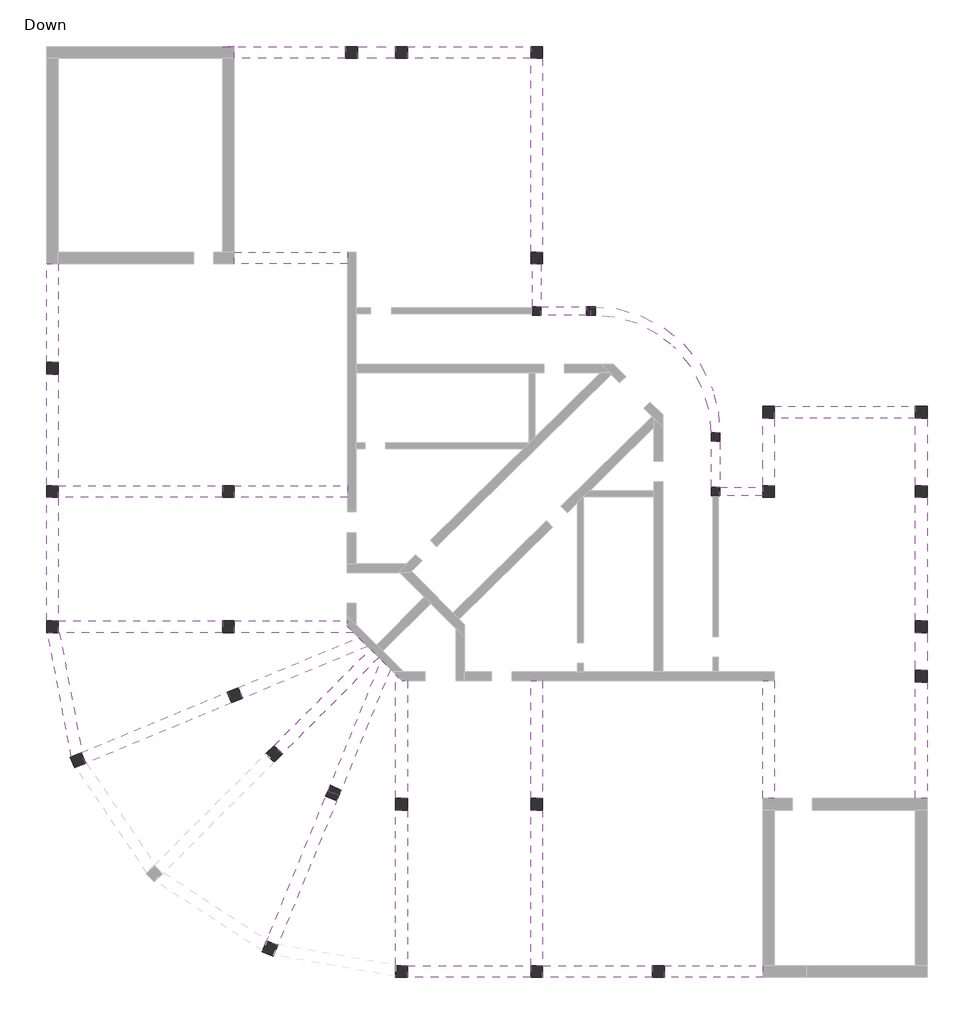
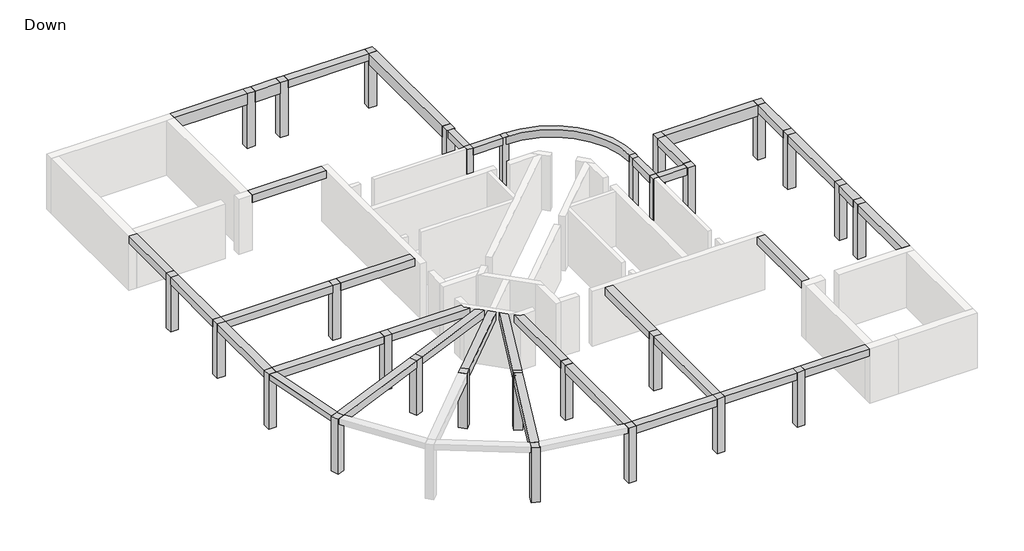
# One storey, part 2 of 2: 37 beams, 29 columns.
# Revit data of these elements (continued)
# Element 42 (IfcColumn, "Concrete Rectengular Column : 40/40") (continued)
#   Phase Created = New Construction
#   Materials on its faces: "Concrete"
# Element 43 (IfcColumn, "Concrete Rectengular Column : 40/40")
#   Comments = ""
#   Mark = "C6"
#   SOFiSTiK_AMG_Comments = ""
#   SOFiSTiK_AMG_Scheduled = yes
#   SOFiSTiK_AMG_Adjusted = yes
#   Structural Material = Concrete
#   Phase Created = New Construction
#   Materials on its faces: "Concrete"
# Element 44 (IfcColumn, "Concrete Rectengular Column : 40/40")
#   Comments = ""
#   Mark = "C7"
#   SOFiSTiK_AMG_Comments = ""
#   SOFiSTiK_AMG_Scheduled = yes
#   SOFiSTiK_AMG_Adjusted = yes
#   Structural Material = Concrete
#   Phase Created = New Construction
#   Materials on its faces: "Concrete"
# Element 45 (IfcColumn, "Concrete Rectengular Column : 40/40")
#   Comments = ""
#   Mark = "C8"
#   SOFiSTiK_AMG_Comments = ""
#   SOFiSTiK_AMG_Scheduled = yes
#   SOFiSTiK_AMG_Adjusted = yes
#   Structural Material = Concrete
#   Phase Created = New Construction
#   Materials on its faces: "Concrete"
# Element 46 (IfcColumn, "Concrete Rectengular Column : 40/40")
#   Comments = ""
#   Mark = "C9"
#   SOFiSTiK_AMG_Comments = ""
#   SOFiSTiK_AMG_Scheduled = yes
#   SOFiSTiK_AMG_Adjusted = yes
#   Structural Material = Concrete
#   Phase Created = New Construction
#   Materials on its faces: "Concrete"
# Element 47 (IfcColumn, "Concrete Rectengular Column : 40/40")
#   Comments = ""
#   Mark = "C10"
#   SOFiSTiK_AMG_Comments = ""
#   SOFiSTiK_AMG_Scheduled = yes
#   SOFiSTiK_AMG_Adjusted = yes
#   Structural Material = Concrete
#   Phase Created = New Construction
#   Materials on its faces: "Concrete"
# Element 48 (IfcColumn, "Concrete Rectengular Column : 40/40")
#   Comments = ""
#   Mark = "C11"
#   SOFiSTiK_AMG_Comments = ""
#   SOFiSTiK_AMG_Scheduled = yes
#   SOFiSTiK_AMG_Adjusted = yes
#   Structural Material = Concrete
#   Phase Created = New Construction
#   Materials on its faces: "Concrete"
# Element 49 (IfcColumn, "Concrete Rectengular Column : 40/40")
#   Comments = ""
#   Mark = "C12"
#   SOFiSTiK_AMG_Comments = ""
#   SOFiSTiK_AMG_Scheduled = yes
#   SOFiSTiK_AMG_Adjusted = yes
#   Structural Material = Concrete
#   Phase Created = New Construction
#   Materials on its faces: "Concrete"
# Element 50 (IfcColumn, "Concrete Rectengular Column : 40/40")
#   Comments = ""
#   Mark = "C13"
#   SOFiSTiK_AMG_Comments = ""
#   SOFiSTiK_AMG_Scheduled = yes
#   SOFiSTiK_AMG_Adjusted = yes
#   Structural Material = Concrete
#   Phase Created = New Construction
#   Materials on its faces: "Concrete"
# Element 51 (IfcColumn, "Concrete Rectengular Column : 40/40")
#   Comments = ""
#   Mark = "C14"
#   SOFiSTiK_AMG_Comments = ""
#   SOFiSTiK_AMG_Scheduled = yes
#   SOFiSTiK_AMG_Adjusted = yes
#   Structural Material = Concrete
#   Phase Created = New Construction
#   Materials on its faces: "Concrete"
# Element 52 (IfcColumn, "Concrete Rectengular Column : 40/40")
#   Comments = ""
#   Mark = "C15"
#   SOFiSTiK_AMG_Comments = ""
#   SOFiSTiK_AMG_Scheduled = yes
#   SOFiSTiK_AMG_Adjusted = yes
#   Structural Material = Concrete
#   Phase Created = New Construction
#   Materials on its faces: "Concrete"
# Element 53 (IfcColumn, "Concrete Rectengular Column : 40/40")
#   Comments = ""
#   Mark = "C16"
#   SOFiSTiK_AMG_Comments = ""
#   SOFiSTiK_AMG_Scheduled = yes
#   SOFiSTiK_AMG_Adjusted = yes
#   Structural Material = Concrete
#   Phase Created = New Construction
#   Materials on its faces: "Concrete"
# Element 54 (IfcColumn, "Concrete Rectengular Column : 40/40")
#   Comments = ""
#   Mark = "C18"
#   SOFiSTiK_AMG_Comments = ""
#   SOFiSTiK_AMG_Scheduled = yes
#   SOFiSTiK_AMG_Adjusted = yes
#   Structural Material = Concrete
#   Phase Created = New Construction
#   Materials on its faces: "Concrete"
# Element 55 (IfcColumn, "Concrete Rectengular Column : 40/40")
#   Comments = ""
#   Mark = "C19"
#   SOFiSTiK_AMG_Comments = ""
#   SOFiSTiK_AMG_Scheduled = yes
#   SOFiSTiK_AMG_Adjusted = yes
#   Structural Material = Concrete
#   Phase Created = New Construction
#   Materials on its faces: "Concrete"
# Element 56 (IfcColumn, "Concrete Rectengular Column : 40/40")
#   Comments = ""
#   Mark = "C20"
#   SOFiSTiK_AMG_Comments = ""
#   SOFiSTiK_AMG_Scheduled = yes
#   SOFiSTiK_AMG_Adjusted = yes
#   Structural Material = Concrete
#   Phase Created = New Construction
#   Materials on its faces: "Concrete"
# Element 57 (IfcColumn, "Concrete Rectengular Column : 40/40")
#   Comments = ""
#   Mark = "C21"
#   SOFiSTiK_AMG_Comments = ""
#   SOFiSTiK_AMG_Scheduled = yes
#   SOFiSTiK_AMG_Adjusted = yes
#   Structural Material = Concrete
#   Phase Created = New Construction
#   Materials on its faces: "Concrete"
# Element 58 (IfcColumn, "Concrete Rectengular Column : 40/40")
#   Comments = ""
#   Mark = "C22"
#   SOFiSTiK_AMG_Comments = ""
#   SOFiSTiK_AMG_Scheduled = yes
#   SOFiSTiK_AMG_Adjusted = yes
#   Structural Material = Concrete
#   Phase Created = New Construction
#   Materials on its faces: "Concrete"
# Element 59 (IfcColumn, "Concrete Rectengular Column : 40/40")
#   Comments = ""
#   Mark = "C23"
#   SOFiSTiK_AMG_Comments = ""
#   SOFiSTiK_AMG_Scheduled = yes
#   SOFiSTiK_AMG_Adjusted = yes
#   Structural Material = Concrete
#   Phase Created = New Construction
#   Materials on its faces: "Concrete"
# Element 60 (IfcColumn, "Concrete Rectengular Column : 40/40")
#   Comments = ""
#   Mark = "C24"
#   SOFiSTiK_AMG_Comments = ""
#   SOFiSTiK_AMG_Scheduled = yes
#   SOFiSTiK_AMG_Adjusted = yes
#   Structural Material = Concrete
#   Phase Created = New Construction
#   Materials on its faces: "Concrete"
# Element 61 (IfcColumn, "Concrete Rectengular Column : 40/40")
#   Comments = ""
#   Mark = "C25"
#   SOFiSTiK_AMG_Comments = ""
#   SOFiSTiK_AMG_Scheduled = yes
#   SOFiSTiK_AMG_Adjusted = yes
#   Structural Material = Concrete
#   Phase Created = New Construction
#   Materials on its faces: "Concrete"
# Element 62 (IfcColumn, "Concrete Rectengular Column : 40/40")
#   Comments = ""
#   Mark = "C26"
#   SOFiSTiK_AMG_Comments = ""
#   SOFiSTiK_AMG_Scheduled = yes
#   SOFiSTiK_AMG_Adjusted = yes
#   Structural Material = Concrete
#   Phase Created = New Construction
#   Materials on its faces: "Concrete"
# Element 63 (IfcColumn, "Concrete Rectengular Column : 40/40")
#   Comments = ""
#   Mark = "C27"
#   SOFiSTiK_AMG_Comments = ""
#   SOFiSTiK_AMG_Scheduled = yes
#   SOFiSTiK_AMG_Adjusted = yes
#   Structural Material = Concrete
#   Phase Created = New Construction
#   Materials on its faces: "Concrete"
# Element 64 (IfcColumn, "Concrete Rectengular Column : 40/40")
#   Comments = ""
#   Mark = "C28"
#   SOFiSTiK_AMG_Comments = ""
#   SOFiSTiK_AMG_Scheduled = yes
#   SOFiSTiK_AMG_Adjusted = yes
#   Structural Material = Concrete
#   Phase Created = New Construction
#   Materials on its faces: "Concrete"
# Element 65 (IfcColumn, "Concrete Rectengular Column : 40/40")
#   Comments = ""
#   Mark = "C29"
#   SOFiSTiK_AMG_Comments = ""
#   SOFiSTiK_AMG_Scheduled = yes
#   SOFiSTiK_AMG_Adjusted = yes
#   Structural Material = Concrete
#   Phase Created = New Construction
#   Materials on its faces: "Concrete"
# Element 66 (IfcColumn, "Concrete Rectengular Column : 40/40")
#   Comments = ""
#   Mark = "C30"
#   SOFiSTiK_AMG_Comments = ""
#   SOFiSTiK_AMG_Scheduled = yes
#   SOFiSTiK_AMG_Adjusted = yes
#   Structural Material = Concrete
#   Phase Created = New Construction
#   Materials on its faces: "Concrete"
# Materials
#   "Concrete": class "Concrete", colour RGB 192 192 192, transparency 0, Keynote = "01000", Description = "Cast-in-place concrete", Cost = 0
